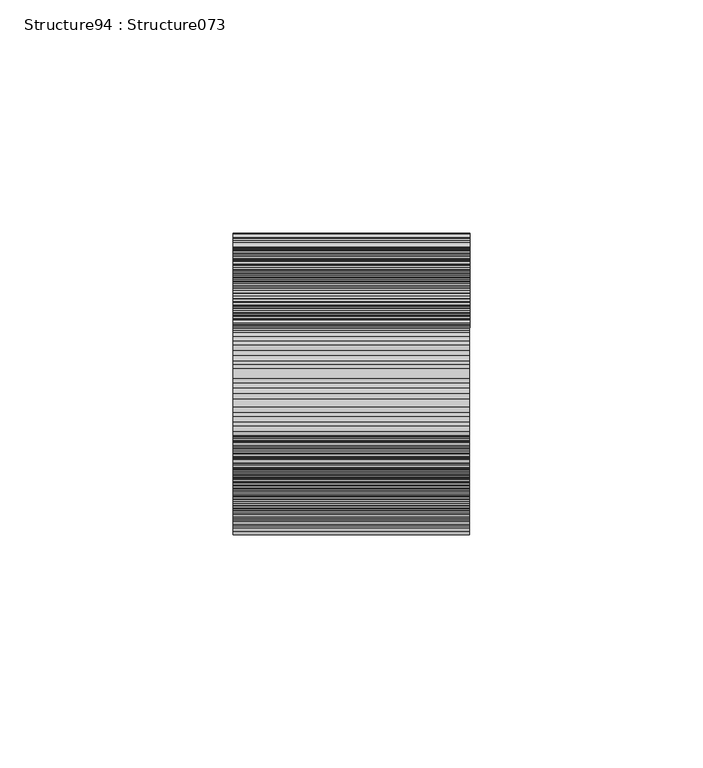
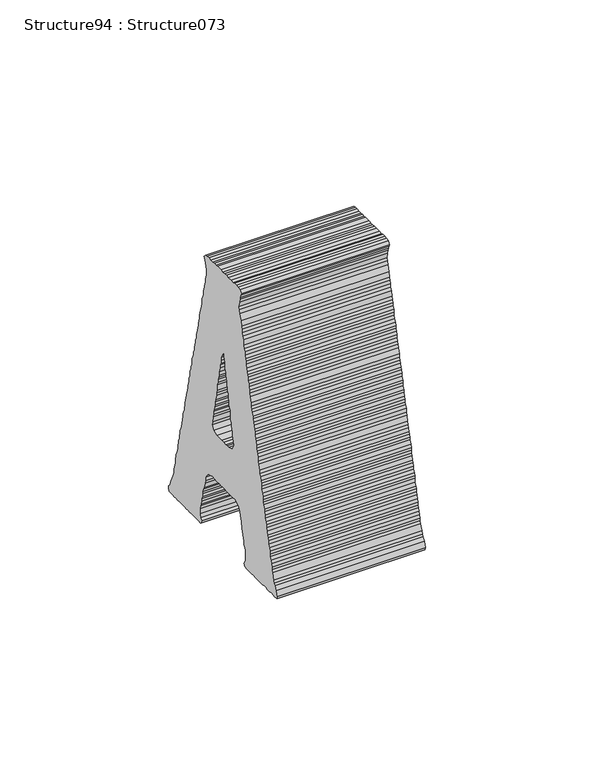
"""IFC4 building model written with IfcOpenShell, lengths in millimetres: proxy geometry, Structure94 : Structure073."""

from ifc_helpers import new_model, si_unit, frame, origin, place, context, project, spatial, polyline, outline, extrude, source, transform, mapped, element, save


def structure94_structure073_8799ebab(model_context):
    return source(origin(), model_context, "Body", "SweptSolid", [
        extrude(outline(polyline([(0.9094651, 0.0), (2.0811665, -0.5191353), (2.9906316, -0.6525662), (4.1562841, -0.7810157), (5.1991801, -1.1663641), (5.9748585, -1.299795), (7.1504738, -1.690125), (8.1894559, -1.690125), (9.3551083, -2.0808107), (10.2645735, -2.3426912), (11.4362748, -2.5995901), (12.3453841, -2.8564891), (13.3818755, -2.9849386), (14.1582655, -3.3756243), (15.4626861, -3.5090552), (16.3721513, -3.5090552), (17.5385154, -3.7709356), (19.491944, -4.4131831), (20.2718921, -4.6750635), (21.3101626, -4.9369439), (22.3470097, -4.9369439), (23.2561191, -5.1991802), (24.4278204, -5.5895101), (25.4700048, -5.9748585), (26.6363689, -5.9748585), (27.4124031, -6.3651885), (28.7175354, -6.6270688), (30.535754, -7.0177546), (31.5743802, -7.1462041), (32.7400327, -7.4080845), (33.6555467, -7.7934329), (35.4741211, -7.7934329), (36.5102567, -7.536534), (37.5492387, -7.279635), (38.3288311, -6.8843236), (39.3671015, -6.3651885), (40.4099976, -7.279635), (40.5395145, -8.1837629), (40.5395145, -9.0982094), (40.2826155, -10.2645735), (40.2826155, -11.3021323), (40.5395145, -12.4734779), (40.4099976, -13.2541376), (40.5395145, -14.1636028), (40.5395145, -16.2390762), (40.2826155, -17.2819723), (40.2826155, -18.3198869), (40.5395145, -19.4858951), (40.4099976, -20.6622221), (40.4099976, -22.3473656), (40.2826155, -23.5187111), (40.5395145, -24.422839), (40.5395145, -25.599166), (40.4099976, -26.5036497), (40.2826155, -27.669658), (39.2382962, -28.455655), (38.3288311, -27.9315384), (37.4197218, -27.669658), (36.6397736, -27.5461899), (35.4741211, -27.2843095), (33.5199809, -26.8939796), (32.6112274, -27.15586), (31.4448633, -27.4177404), (29.3636968, -28.1937747), (27.545834, -28.455655), (26.5089869, -28.712554), (25.3372855, -28.8459849), (24.2943895, -29.1078654), (23.2561191, -29.6216633), (21.3101626, -29.7504686), (20.2718921, -30.012349), (19.491944, -30.5361099), (18.3202426, -30.5361099), (17.2816164, -30.9214583), (16.3721513, -31.1783574), (15.3356599, -31.1783574), (14.1582655, -31.4405936), (13.1253323, -31.8309234), (12.2158672, -32.2212534), (11.4362748, -32.3546843), (10.2645735, -32.4831338), (9.3551083, -32.8684823), (8.1894559, -32.8684823), (7.1504738, -33.259168), (6.2374505, -33.3925989), (5.0714422, -33.6494979), (3.2475306, -34.2967268), (2.0811665, -34.2967268), (1.1720572, -34.5586072), (0.1334309, -34.8208435), (-1.0382704, -35.3396228), (-1.8178628, -35.4730537), (-2.8568449, -35.7299528), (-3.8990293, -35.8633837), (-5.0653934, -36.2487321), (-5.8471206, -36.5109684), (-7.0166871, -36.5109684), (-8.1826954, -36.9012983), (-8.9644226, -37.0297478), (-10.1364798, -37.4200777), (-11.1690572, -37.5535086), (-12.2115974, -37.6769767), (-12.9915456, -37.9388571), (-14.03373, -38.3295427), (-15.3292552, -38.4579923), (-16.3678815, -38.7198727), (-18.1861001, -39.1102026), (-19.3581573, -39.3671016), (-20.2672666, -39.7577873), (-21.4371888, -40.0196677), (-22.2189161, -40.2765667), (-23.1223323, -40.5384471), (-24.1648726, -40.5384471), (-25.465735, -41.0522451), (-26.5025822, -41.3144814), (-27.4173846, -41.4479123), (-28.4560108, -41.4479123), (-29.235959, -41.7048112), (-30.5311284, -42.0951412), (-31.3110766, -42.2285721), (-32.3536168, -42.6139205), (-33.5214042, -42.6139205), (-34.4308693, -43.1330558), (-35.3399786, -43.3949362), (-36.37647, -43.3949362), (-37.5424783, -43.6568165), (-38.7202285, -44.0471465), (-39.6236447, -44.3040455), (-40.405372, -44.5613002), (-41.5752942, -44.6947312), (-42.6139205, -45.0850611), (-43.7856218, -45.3469415), (-44.8221132, -45.3469415), (-45.7372714, -45.475391), (-46.6406876, -45.9941704), (-47.812389, -46.2514252), (-48.8510152, -46.5133056), (-49.7601245, -46.5133056), (-50.6731478, -46.9036355), (-52.8777823, -47.5508644), (-53.7929405, -47.9415501), (-54.5689747, -48.33188), (-55.738897, -49.1125398), (-57.5532016, -49.7601246), (-58.4665807, -49.4982442), (-58.5957419, -48.2034305), (-58.4665807, -47.4273963), (-58.3331498, -46.2514252), (-58.5957419, -45.2135106), (-58.5957419, -44.0471465), (-58.3331498, -43.0046063), (-58.3331498, -42.0951412), (-58.4665807, -41.0522451), (-58.4665807, -40.1481172), (-58.5957419, -38.8483222), (-58.5957419, -37.9388571), (-58.4665807, -36.9012983), (-58.3331498, -35.7299528), (-58.5957419, -34.8208435), (-58.5957419, -31.8309234), (-58.3331498, -30.6645593), (-57.4297336, -30.1407986), (-56.6480063, -30.5361099), (-55.6115149, -30.7930088), (-53.3972734, -30.7930088), (-52.3586471, -30.7930088), (-51.4495378, -30.5361099), (-50.6731478, -30.1407986), (-49.3683714, -30.012349), (-48.4592621, -29.7504686), (-47.5497969, -29.3597829), (-46.6406876, -29.1078654), (-45.6038405, -28.8459849), (-43.2661308, -28.5841045), (-41.5752942, -27.9315384), (-40.2762109, -27.669658), (-38.9767716, -27.0274105), (-38.1950444, -26.1129639), (-37.4190102, -24.6847195), (-37.6759092, -23.6471607), (-37.6759092, -21.5667058), (-37.5424783, -20.2669108), (-37.5424783, -17.5438527), (-37.6759092, -16.3675257), (-37.4190102, -15.4633978), (-37.5424783, -14.4205018), (-37.6759092, -13.3829429), (-37.5424783, -12.4734779), (-37.4190102, -11.1736828), (-37.6759092, -10.393023), (-38.0676623, -8.8363291), (-38.8476105, -8.0553134), (-40.2762109, -7.0177546), (-41.4422191, -7.0177546), (-42.6139205, -6.7558741), (-44.561656, -6.236739), (-45.3472973, -5.7179595), (-46.5133056, -5.4560792), (-47.2932538, -5.3276297), (-48.33188, -5.3276297), (-49.3683714, -4.8084944), (-50.4126907, -4.6750635), (-51.4495378, -4.546614), (-52.3586471, -4.1612656), (-53.6595096, -3.7709356), (-55.3489229, -3.8993851), (-56.6480063, -4.2897151), (-57.2966585, -4.9369439), (-58.5957419, -4.1612656), (-58.4665807, -2.9849386), (-58.3331498, -1.9473798), (-58.3331498, 0.1284494), (-58.4665807, 1.1660082), (-58.4665807, 2.2089042), (-58.3331498, 3.1180136), (-58.4665807, 4.0324601), (-58.4665807, 5.3272738), (-58.3331498, 6.1029522), (-58.4665807, 7.4027472), (-58.3331498, 8.1837628), (-58.5957419, 9.2213216), (-58.3331498, 10.3976485), (-58.5957419, 11.5640127), (-58.4665807, 12.473122), (-58.3331498, 13.516018), (-58.3331498, 14.5485954), (-57.2966585, 14.9442625), (-56.3875492, 14.6820263), (-55.738897, 14.0298159), (-54.5689747, 13.772917), (-53.7929405, 13.382587), (-52.6151903, 12.8634519), (-50.6731478, 11.9543426), (-49.8875066, 11.6924622), (-48.5941162, 11.5640127), (-47.5497969, 11.3017764), (-46.6406876, 11.0448774), (-45.8646534, 10.6545476), (-44.5616561, 10.526098), (-42.6139205, 10.2642176), (-41.4422191, 9.8738877), (-40.5384471, 9.483202), (-39.6236447, 9.2213216), (-38.4576364, 9.0928721), (-37.4190102, 8.969404), (-36.5059869, 8.8359731), (-35.6004358, 8.3171937), (-34.2956593, 8.1837628), (-33.3922431, 8.0549575), (-32.3536168, 7.926508), (-31.4405935, 7.5361781), (-30.4019673, 7.1458482), (-29.235959, 6.8889491), (-27.5447666, 6.6270687), (-26.3752002, 6.2363831), (-25.203143, 6.1029522), (-24.4235506, 5.8460531), (-23.3849244, 5.4607047), (-22.4793732, 5.3272738), (-21.3037579, 4.9369438), (-20.2672666, 4.9369438), (-19.3581573, 4.6747076), (-18.319531, 4.4178086), (-17.1474738, 4.1559282), (-15.2018732, 3.6371488), (-14.1632469, 3.3802498), (-13.1207067, 3.3802498), (-12.2115974, 2.9895641), (-11.3024881, 2.5992342), (-10.0012698, 2.5992342), (-9.2270147, 2.0804548), (-8.1826954, 2.0804548), (-7.0166871, 1.9520053), (-5.9745027, 1.4278887), (-5.0653934, 1.4278887), (-4.1619771, 0.9091093), (-2.8568449, 0.7756784), (-1.9473797, 0.7756784), (-0.7817273, 0.2618803), (0.0, 0.0), (0.9094651, 0.0)]), holes=[polyline([(-20.9137838, -13.9017224), (-20.9137838, -16.8916423), (-20.7903157, -18.0576507), (-21.0472147, -19.2289962), (-20.7903157, -20.1384613), (-20.9137838, -21.0475706), (-20.2672666, -22.9945945), (-18.5817672, -23.6471607), (-17.2809048, -23.3852802), (-16.3678815, -23.1280254), (-15.4623303, -22.866145), (-14.1632469, -22.9945945), (-13.2480888, -22.4807965), (-12.2115974, -22.3473656), (-11.3024881, -22.2189161), (-10.393023, -21.8285863), (-9.3508386, -21.6951553), (-8.3122123, -21.6951553), (-7.146204, -21.5667058), (-6.3644768, -21.1760201), (-5.3276296, -20.9191211), (-4.2854452, -20.9191211), (-3.117302, -20.4003417), (-1.9473797, -20.4003417), (-1.0382704, -20.0100118), (-0.2561874, -19.8765809), (1.0389821, -19.7477755), (2.0811665, -19.4858951), (3.1180136, -19.2289962), (4.0274787, -19.1005467), (5.0714422, -19.1005467), (6.1082894, -18.5817673), (7.0177545, -18.4483364), (8.1894559, -18.4483364), (9.2216774, -18.0576507), (10.1368356, -17.7957702), (11.0463007, -17.7957702), (10.1368356, -17.1535228), (9.0928721, -16.7582114), (8.056025, -16.6297619), (6.8900167, -16.6297619), (6.1082894, -16.1106267), (4.9365881, -15.9771958), (3.1180136, -15.4633978), (1.8189302, -15.3299669), (0.9094651, -15.2015174), (0.0, -14.939637), (-1.0382704, -14.8108317), (-2.2078369, -14.4205018), (-4.2854452, -14.2870708), (-5.3276296, -14.0351533), (-6.3644768, -13.9017224), (-8.1826954, -13.5113925), (-9.2270147, -12.9922573), (-10.2638619, -12.9922573), (-11.1690572, -12.7303769), (-12.3446725, -12.6019274), (-13.1207067, -12.2165788), (-14.286715, -12.2165788), (-15.4623303, -11.8212676), (-17.2809048, -11.5640128), (-18.5817672, -11.3021323), (-20.1377496, -12.0831479), (-20.9137838, -13.9017224)])]), frame((-56111.641531, 291007.8168109, -317.0048136), z_axis=(-0.9999998917542984, 0.00046528635450596156, 0.0), x_axis=(0.0, 0.0, 1.0)), (0.0, 0.0, 1.0), 50.8),
    ])


if __name__ == "__main__":
    model = new_model("IFC4")
    model_context = context("Model", 3, world=origin())
    ifc_project = project(units=[si_unit("LENGTHUNIT", "METRE", prefix="MILLI")], contexts=[model_context])
    site = spatial("IfcSite", under=ifc_project)
    building = spatial("IfcBuilding", under=site)
    placement = place(None, origin())
    structure94_structure073_shape = structure94_structure073_8799ebab(model_context)
    element("IfcBuildingElementProxy", 1, Name="Structure94 : Structure073", ObjectType="Structure94 : Structure073", at=placement, inside=building, context=model_context, shape_type="MappedRepresentation", body=[
        mapped(structure94_structure073_shape, transform((0.0, 0.0, 0.0), x_axis=(1.0, 0.0, 0.0), y_axis=(0.0, 1.0, 0.0), z_axis=(0.0, 0.0, 1.0))),
    ])
    save(model, "model.ifc")

# Revit data of these elements
# Type "Structure94 : Structure073"
#   NameOverride = "Structure073"
# Element 1 (IfcBuildingElementProxy, "Structure94 : Structure073")
#   Materials on its faces: "BRUSHED ALUMINUM LETTERING"
# Materials
#   "BRUSHED ALUMINUM LETTERING": class "Unassigned", colour RGB 169 181 186, transparency 0, Cost = 0
